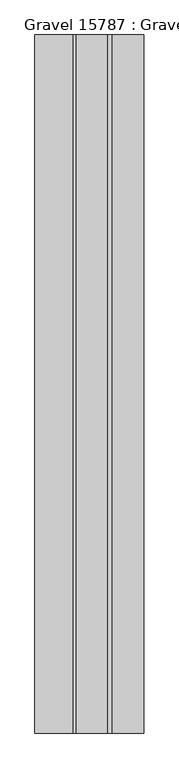
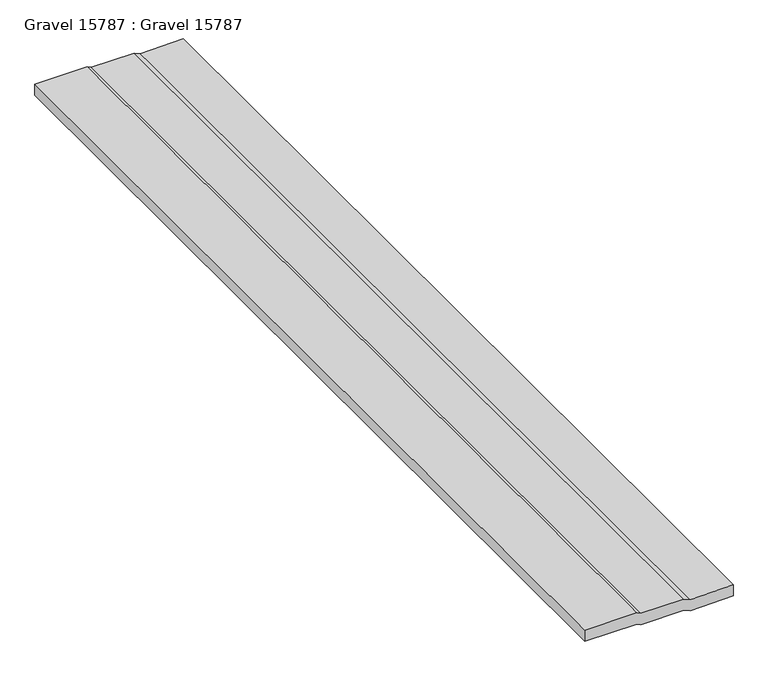
"""IFC4 building model written with IfcOpenShell, lengths in millimetres: proxy geometry, Gravel 15787 : Gravel 15787."""

from ifc_helpers import new_model, si_unit, frame, origin, place, context, project, spatial, polyline, outline, extrude, source, transform, mapped, element, save


def gravel_15787_gravel_15787_052f081c(model_context):
    return source(origin(), model_context, "Body", "SweptSolid", [
        extrude(outline(polyline([(40274.2359464, -4902.3767758), (40269.9546964, -4893.6663265), (40269.9546964, -4803.0794125), (40264.2272344, -4790.2347731), (40265.8726651, -4699.8063764), (40290.6109464, -4699.8063764), (40288.9655157, -4790.2347731), (40294.6929777, -4803.0794125), (40294.6929777, -4893.6663265), (40298.9742277, -4902.3767758), (40298.9742277, -5011.8762875), (40274.2359464, -5011.8762875), (40274.2359464, -4902.3767758)])), frame((0.0, -1052.6406573, 0.0), z_axis=(0.0, 1.0, 0.0), x_axis=(0.0, 0.0, 1.0)), (0.0, 0.0, 1.0), 2000.0),
    ])


if __name__ == "__main__":
    model = new_model("IFC4")
    model_context = context("Model", 3, world=origin())
    ifc_project = project(units=[si_unit("LENGTHUNIT", "METRE", prefix="MILLI")], contexts=[model_context])
    site = spatial("IfcSite", under=ifc_project)
    building = spatial("IfcBuilding", under=site)
    placement = place(None, origin())
    gravel_15787_gravel_15787_shape = gravel_15787_gravel_15787_052f081c(model_context)
    element("IfcBuildingElementProxy", 1, Name="Gravel 15787 : Gravel 15787", ObjectType="Gravel 15787 : Gravel 15787", at=placement, inside=building, context=model_context, shape_type="MappedRepresentation", body=[
        mapped(gravel_15787_gravel_15787_shape, transform((0.0, 0.0, 0.0), x_axis=(1.0, 0.0, 0.0), y_axis=(0.0, 1.0, 0.0), z_axis=(0.0, 0.0, 1.0))),
    ])
    save(model, "model.ifc")

# Revit data of these elements
# Type "Gravel 15787 : Gravel 15787"
#   NameOverride = "Gravel"
# Element 1 (IfcBuildingElementProxy, "Gravel 15787 : Gravel 15787")
#   Materials on its faces: "GRAVEL BALLAST"
# Materials
#   "GRAVEL BALLAST": class "Unassigned", colour RGB 128 128 128, transparency 0, Cost = 0
